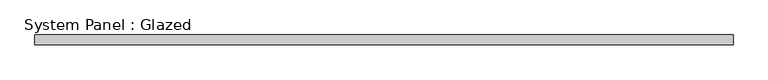
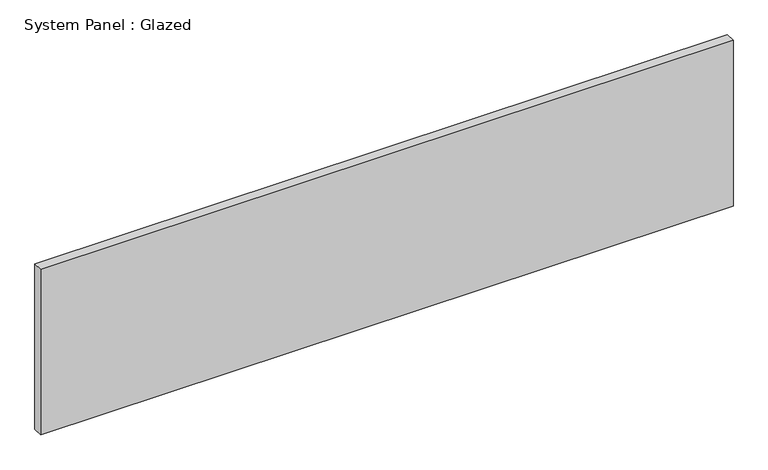
"""IFC4 building model written with IfcOpenShell, lengths in millimetres: plate geometry, System Panel : Glazed."""

from ifc_helpers import new_model, si_unit, origin, origin_with_axes, place, context, project, spatial, polyline, outline, extrude, source, transform, mapped, element, save


def system_panel_glazed_1da98b3e(model_context):
    return source(origin(), model_context, "Body", "SweptSolid", [
        extrude(outline(polyline([(890.0, -49.5), (-890.0, -49.5), (-890.0, -24.5), (890.0, -24.5), (890.0, -49.5)])), origin_with_axes(), (0.0, 0.0, 1.0), 450.0),
    ])


if __name__ == "__main__":
    model = new_model("IFC4")
    model_context = context("Model", 3, world=origin())
    ifc_project = project(units=[si_unit("LENGTHUNIT", "METRE", prefix="MILLI")], contexts=[model_context])
    site = spatial("IfcSite", under=ifc_project)
    building = spatial("IfcBuilding", under=site)
    placement = place(None, origin())
    system_panel_glazed_shape = system_panel_glazed_1da98b3e(model_context)
    element("IfcPlate", 1, ObjectType="System Panel : Glazed", at=placement, inside=building, context=model_context, shape_type="MappedRepresentation", body=[
        mapped(system_panel_glazed_shape, transform((0.0, 0.0, 0.0), x_axis=(1.0, 0.0, 0.0), y_axis=(0.0, 1.0, 0.0), z_axis=(0.0, 0.0, 1.0))),
    ])
    save(model, "model.ifc")

# Revit data of these elements
# Type "System Panel : Glazed"
#   Keynote = "H11"
#   Construction Type Id = "GSP4R"
#   Analytic Construction = "1/8 in Pilkington single glazing"
#   Visual Light Transmittance = 0.9
#   Solar Heat Gain Coefficient = 0.86
#   Heat Transfer Coefficient (U) = 6.7069 W/(m²·K)
# Element 1 (IfcPlate, "System Panel : Glazed")
#   Materials on its faces: "Glass"
# Materials
#   "Glass": class "Glass", colour RGB 0 128 192, transparency 0.9, Description = "Soda Lime Glass", Cost = 0
